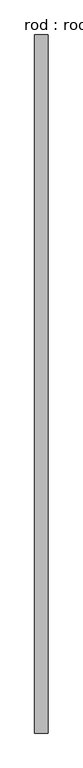
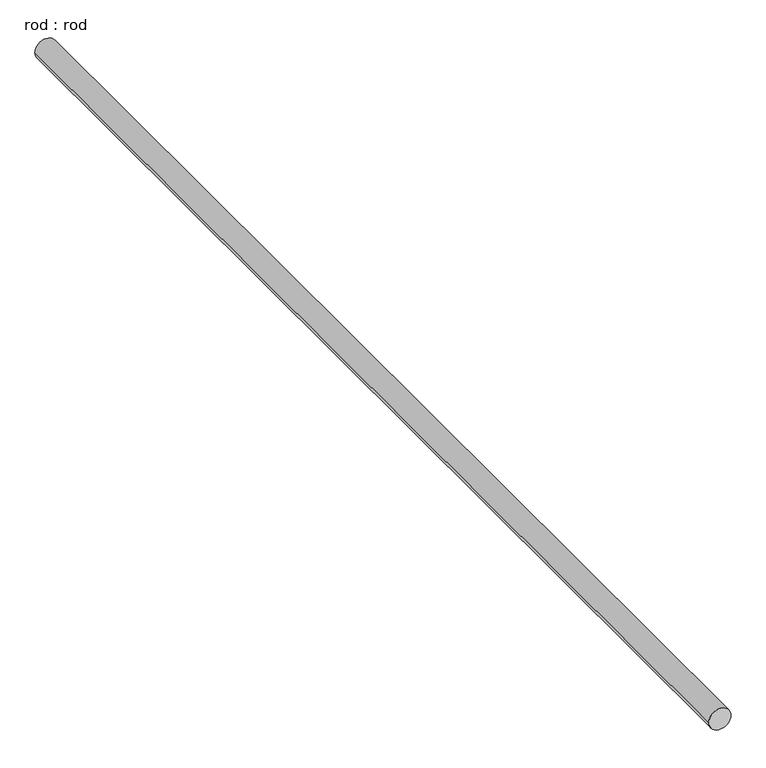
"""IFC4 building model written with IfcOpenShell, lengths in millimetres: proxy geometry, rod : rod."""

import ifcopenshell
import ifcopenshell.guid

model = None  # the IFC model being written
_history = None  # IfcOwnerHistory: only IFC2X3 demands one
_inside = {}  # id of a spatial element -> (the spatial element, [elements in it])
_under = {}  # id of a project, library or spatial element -> (it, [spatial elements below it])
_declared = {}  # id of a project -> (the project, [libraries it declares])
_typed = {}  # id of a type object -> (the type object, [elements of that type])
_made_of = {}  # id of a material, layer set ... -> (it, [elements and type objects made of it])


def new_model(schema):
    """Start an empty IFC model of exactly this schema.

    Asked for "IFC4X3", IfcOpenShell would pick the latest addendum, in which some entities
    have other attributes; the version numbers below select the first issue.
    IFC2X3 requires an IfcOwnerHistory on every rooted entity: one is made here for all.
    """
    global model, _history
    if schema == "IFC4X3":
        model = ifcopenshell.file(schema_version=(4, 3, 0, 0))
    else:
        model = ifcopenshell.file(schema=schema)
    _inside.clear()
    _under.clear()
    _declared.clear()
    _typed.clear()
    _made_of.clear()
    _history = None
    if model.schema == "IFC2X3":
        org = make("IfcOrganization", Name="unknown")
        user = make(
            "IfcPersonAndOrganization",
            ThePerson=make("IfcPerson", FamilyName="unknown"),
            TheOrganization=org,
        )
        app = make(
            "IfcApplication",
            ApplicationDeveloper=org,
            Version="unknown",
            ApplicationFullName="unknown",
            ApplicationIdentifier="unknown",
        )
        _history = make(
            "IfcOwnerHistory",
            OwningUser=user,
            OwningApplication=app,
            ChangeAction="ADDED",
            CreationDate=0,
        )
    return model


def make(cls, **values):
    """One entity of the class cls with the attributes given. An attribute that is None is left unset."""
    return model.create_entity(
        cls, **{name: value for name, value in values.items() if value is not None}
    )


def rooted(cls, **values):
    """An entity with a GlobalId (a new one), such as an element, a storey or a relation."""
    return make(cls, GlobalId=ifcopenshell.guid.new(), OwnerHistory=_history, **values)


def si_unit(unit_type, name, prefix=None):
    """IfcSIUnit, for example si_unit("LENGTHUNIT", "METRE", prefix="MILLI")."""
    return make("IfcSIUnit", UnitType=unit_type, Prefix=prefix, Name=name)


def assignment(units):
    """IfcUnitAssignment: the units of a project."""
    return None if units is None else make("IfcUnitAssignment", Units=units)


def point(xyz):
    """IfcCartesianPoint."""
    return None if xyz is None else make("IfcCartesianPoint", Coordinates=xyz)


def direction(xyz):
    """IfcDirection."""
    return None if xyz is None else make("IfcDirection", DirectionRatios=xyz)


def frame(location, z_axis=None, x_axis=None):
    """IfcAxis2Placement3D, a coordinate frame: its origin and axes. An axis left out is left unset."""
    return make(
        "IfcAxis2Placement3D",
        Location=point(location),
        Axis=direction(z_axis),
        RefDirection=direction(x_axis),
    )


def frame_2d(location, x_axis=None):
    """IfcAxis2Placement2D, a coordinate frame in the plane: its origin and x axis."""
    return make(
        "IfcAxis2Placement2D", Location=point(location), RefDirection=direction(x_axis)
    )


def origin():
    """The frame at (0, 0, 0) with its axes left unset."""
    return frame((0.0, 0.0, 0.0))


def place(relative_to, where):
    """IfcLocalPlacement: puts the frame where relative to a parent placement (None: the world)."""
    return make(
        "IfcLocalPlacement", PlacementRelTo=relative_to, RelativePlacement=where
    )


def context(
    kind, dimensions, precision=None, world=None, true_north=None, identifier=None
):
    """IfcGeometricRepresentationContext, for example the 3D "Model" context."""
    return make(
        "IfcGeometricRepresentationContext",
        ContextIdentifier=identifier,
        ContextType=kind,
        CoordinateSpaceDimension=dimensions,
        Precision=precision,
        WorldCoordinateSystem=world,
        TrueNorth=true_north,
    )


def project(units=None, contexts=None):
    """IfcProject with its units and contexts."""
    return rooted(
        "IfcProject",
        Name="project",
        RepresentationContexts=contexts,
        UnitsInContext=assignment(units),
    )


def spatial(cls, under=None, at=None, **own):
    """A site, building, storey or space (cls), placed at a placement, below another one or the project."""
    s = rooted(cls, ObjectPlacement=at, **own)
    if under is not None:
        _under.setdefault(under.id(), (under, []))[1].append(s)
    return s


def circle_curve(where, radius):
    """IfcCircle in the frame where."""
    return make("IfcCircle", Position=where, Radius=radius)


def trimmed(basis, trim1, trim2, sense, master):
    """IfcTrimmedCurve: the piece of a basis curve between two trims."""
    return make(
        "IfcTrimmedCurve",
        BasisCurve=basis,
        Trim1=trim1,
        Trim2=trim2,
        SenseAgreement=sense,
        MasterRepresentation=master,
    )


def segment(curve, same_sense, transition):
    """IfcCompositeCurveSegment."""
    return make(
        "IfcCompositeCurveSegment",
        Transition=transition,
        SameSense=same_sense,
        ParentCurve=curve,
    )


def composite_curve(segments, self_intersect=None):
    """IfcCompositeCurve: segments joined end to end."""
    return make("IfcCompositeCurve", Segments=segments, SelfIntersect=self_intersect)


def outline(outer, holes=None, kind="AREA"):
    """IfcArbitraryClosedProfileDef: a profile drawn as a closed curve; with holes, ...WithVoids."""
    if holes is None:
        return make("IfcArbitraryClosedProfileDef", ProfileType=kind, OuterCurve=outer)
    return make(
        "IfcArbitraryProfileDefWithVoids",
        ProfileType=kind,
        OuterCurve=outer,
        InnerCurves=holes,
    )


def extrude(swept, where, along, depth):
    """IfcExtrudedAreaSolid: the profile swept, set in the frame where, extruded along a direction by depth."""
    return make(
        "IfcExtrudedAreaSolid",
        SweptArea=swept,
        Position=where,
        ExtrudedDirection=direction(along),
        Depth=depth,
    )


def shape(context_of_items, identifier, shape_type, items):
    """IfcShapeRepresentation: the items that make up one representation, for example the "Body"."""
    return make(
        "IfcShapeRepresentation",
        ContextOfItems=context_of_items,
        RepresentationIdentifier=identifier,
        RepresentationType=shape_type,
        Items=items,
    )


def source(mapping_origin, context_of_items, identifier, shape_type, items):
    """IfcRepresentationMap: a shape defined once, which mapped items show again and again."""
    return make(
        "IfcRepresentationMap",
        MappingOrigin=mapping_origin,
        MappedRepresentation=shape(context_of_items, identifier, shape_type, items),
    )


def transform(
    local_origin,
    x_axis=None,
    y_axis=None,
    z_axis=None,
    scale=None,
    scale2=None,
    scale3=None,
    uniform=True,
):
    """IfcCartesianTransformationOperator3D, or its non-uniform kind. x_axis, y_axis, z_axis: its Axis1, 2, 3."""
    if uniform:
        return make(
            "IfcCartesianTransformationOperator3D",
            Axis1=direction(x_axis),
            Axis2=direction(y_axis),
            LocalOrigin=point(local_origin),
            Scale=scale,
            Axis3=direction(z_axis),
        )
    return make(
        "IfcCartesianTransformationOperator3DnonUniform",
        Axis1=direction(x_axis),
        Axis2=direction(y_axis),
        LocalOrigin=point(local_origin),
        Scale=scale,
        Axis3=direction(z_axis),
        Scale2=scale2,
        Scale3=scale3,
    )


def mapped(mapping_source, mapping_target):
    """IfcMappedItem: shows the shape of a source again, moved by a transform."""
    return make(
        "IfcMappedItem", MappingSource=mapping_source, MappingTarget=mapping_target
    )


def made_of(thing, what):
    """Note that an element or type object is made of a material, layer set ...; save() writes the relation."""
    if what is not None:
        _made_of.setdefault(what.id(), (what, []))[1].append(thing)
    return thing


def element(
    cls,
    number,
    at=None,
    inside=None,
    cuts=None,
    type_object=None,
    material=None,
    context=None,
    identifier="Body",
    shape_type=None,
    held_by="IfcProductDefinitionShape",
    body=None,
    shapes=None,
    **own,
):
    """One element of the class cls, such as IfcWall. Its Tag is "e" and its number.

    at: its placement. inside: the storey or other place that contains it. cuts: it is an
    opening in that element (IfcRelVoidsElement). A single representation is given by context,
    identifier, shape_type and body (its items); several are given by shapes. held_by: the class
    of the entity that holds the representations. save() writes the other relations.
    """
    e = rooted(cls, Tag="e%d" % number, ObjectPlacement=at, **own)
    if body is not None:
        shapes = [shape(context, identifier, shape_type, body)]
    if shapes is not None:
        e.Representation = make(held_by, Representations=shapes)
    if inside is not None:
        _inside.setdefault(inside.id(), (inside, []))[1].append(e)
    if cuts is not None:
        rooted(
            "IfcRelVoidsElement", RelatingBuildingElement=cuts, RelatedOpeningElement=e
        )
    if type_object is not None:
        _typed.setdefault(type_object.id(), (type_object, []))[1].append(e)
    return made_of(e, material)


def aggregate(whole, parts):
    """IfcRelAggregates: a whole, such as a stair, and the parts it consists of."""
    return rooted("IfcRelAggregates", RelatingObject=whole, RelatedObjects=parts)


def save(model, path):
    """Write the relations noted so far, then the file.

    IfcRelAggregates (storeys below a building ...), IfcRelContainedInSpatialStructure (elements
    in a storey), IfcRelDefinesByType, IfcRelAssociatesMaterial and IfcRelDeclares: one each for
    every whole, place, type object, material and project.
    """
    for whole, parts in _under.values():
        aggregate(whole, parts)
    for where, things in _inside.values():
        rooted(
            "IfcRelContainedInSpatialStructure",
            RelatedElements=things,
            RelatingStructure=where,
        )
    for kind, things in _typed.values():
        rooted("IfcRelDefinesByType", RelatedObjects=things, RelatingType=kind)
    for what, things in _made_of.values():
        rooted("IfcRelAssociatesMaterial", RelatedObjects=things, RelatingMaterial=what)
    for by, libraries in _declared.values():
        rooted("IfcRelDeclares", RelatingContext=by, RelatedDefinitions=libraries)
    model.write(path)


def rod_rod_c6a0ea35(model_context):
    return source(origin(), model_context, "Body", "SweptSolid", [
        extrude(outline(composite_curve([segment(trimmed(circle_curve(frame_2d((0.0108462, 0.0)), 200.0), [point((0.0108462, 200.0))], [point((0.0108462, -200.0))], False, "CARTESIAN"), True, "CONTINUOUS"), segment(trimmed(circle_curve(frame_2d((0.0108462, 0.0)), 200.0), [point((0.0108462, -200.0))], [point((0.0108462, 200.0))], False, "CARTESIAN"), True, "CONTINUOUS")], self_intersect=False)), frame((0.0, -6459.0117722, 0.0), z_axis=(0.0, 1.0, 0.0), x_axis=(0.0, 0.0, 1.0)), (0.0, 0.0, 1.0), 21103.4807751),
    ])


if __name__ == "__main__":
    model = new_model("IFC4")
    model_context = context("Model", 3, world=origin())
    ifc_project = project(units=[si_unit("LENGTHUNIT", "METRE", prefix="MILLI")], contexts=[model_context])
    site = spatial("IfcSite", under=ifc_project)
    building = spatial("IfcBuilding", under=site)
    placement = place(None, origin())
    rod_rod_shape = rod_rod_c6a0ea35(model_context)
    element("IfcBuildingElementProxy", 1, Name="rod : rod", ObjectType="rod : rod", at=placement, inside=building, context=model_context, shape_type="MappedRepresentation", body=[
        mapped(rod_rod_shape, transform((0.0, 0.0, 0.0), x_axis=(1.0, 0.0, 0.0), y_axis=(0.0, 1.0, 0.0), z_axis=(0.0, 0.0, 1.0))),
    ])
    save(model, "model.ifc")

# Revit data of these elements
# Type "rod : rod"
#   Default Elevation = 0
